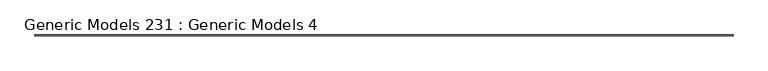
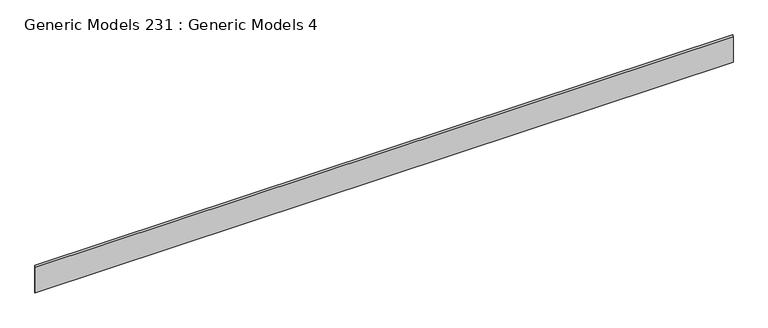
"""IFC4 building model written with IfcOpenShell, lengths in millimetres: proxy geometry, Generic Models 231 : Generic Models 4."""

from ifc_helpers import new_model, si_unit, frame, origin, place, context, project, spatial, polyline, outline, extrude, source, transform, mapped, element, save


def generic_models_231_generic_models_4_fb312406(model_context):
    return source(origin(), model_context, "Body", "SweptSolid", [
        extrude(outline(polyline([(-29179.7896285, 127068.7090401), (-29160.6485041, 127105.9838613), (-29160.6485041, 126342.521), (-29179.7896285, 126342.521), (-29179.7896285, 127068.7090401)])), frame((-20795.7733045, 0.0, 0.0), z_axis=(1.0, 0.0, 0.0), x_axis=(0.0, 1.0, 0.0)), (0.0, 0.0, 1.0), 18643.6),
    ])


if __name__ == "__main__":
    model = new_model("IFC4")
    model_context = context("Model", 3, world=origin())
    ifc_project = project(units=[si_unit("LENGTHUNIT", "METRE", prefix="MILLI")], contexts=[model_context])
    site = spatial("IfcSite", under=ifc_project)
    building = spatial("IfcBuilding", under=site)
    placement = place(None, origin())
    generic_models_231_generic_models_4_shape = generic_models_231_generic_models_4_fb312406(model_context)
    element("IfcBuildingElementProxy", 1, Name="Generic Models 231 : Generic Models 4", ObjectType="Generic Models 231 : Generic Models 4", at=placement, inside=building, context=model_context, shape_type="MappedRepresentation", body=[
        mapped(generic_models_231_generic_models_4_shape, transform((0.0, 0.0, 0.0), x_axis=(1.0, 0.0, 0.0), y_axis=(0.0, 1.0, 0.0), z_axis=(0.0, 0.0, 1.0))),
    ])
    save(model, "model.ifc")

# Revit data of these elements
# Element 1 (IfcBuildingElementProxy, "Generic Models 231 : Generic Models 4")
#   Materials on its faces: "_7/8\" SMOOTH TROWEL EXTERIOR STUCCO (COLOR PER OWNER)"
# Materials
#   "_7/8\" SMOOTH TROWEL EXTERIOR STUCCO (COLOR PER OWNER)": class "Generic", colour RGB 233 233 233, transparency 0, Cost = 0
